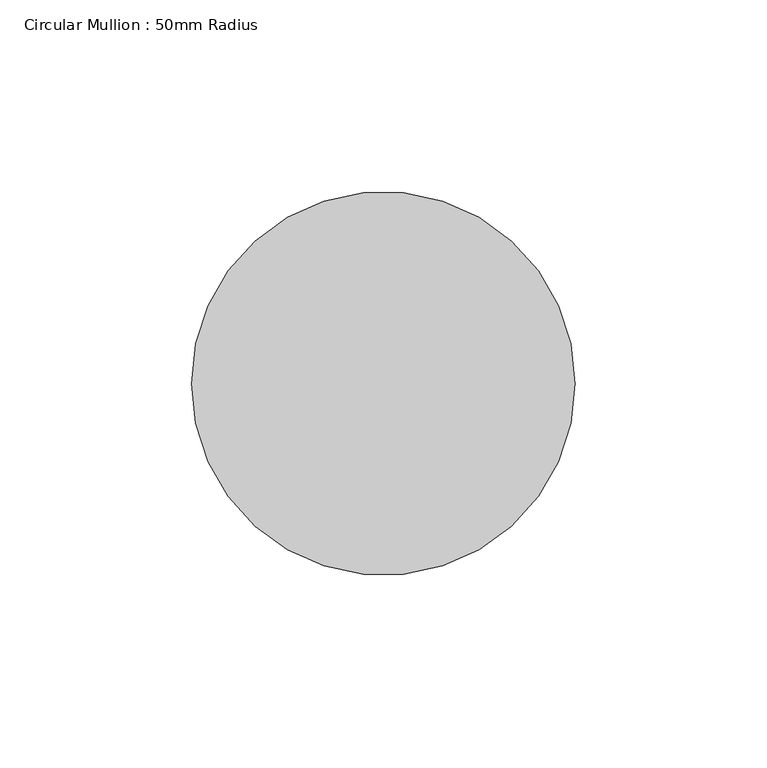
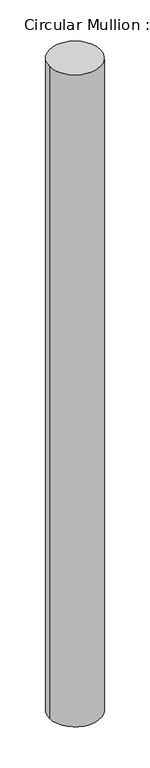
"""IFC4 building model written with IfcOpenShell, lengths in millimetres: member geometry, Circular Mullion : 50mm Radius."""

from ifc_helpers import new_model, si_unit, point, frame, origin, origin_2d, place, context, project, spatial, circle_curve, trimmed, segment, composite_curve, outline, extrude, source, transform, mapped, element, save


def circular_mullion_50mm_radius_b40ed272(model_context):
    return source(origin(), model_context, "Body", "SweptSolid", [
        extrude(outline(composite_curve([segment(trimmed(circle_curve(origin_2d(), 50.0), [point((50.0, 0.0))], [point((-50.0, 0.0))], False, "CARTESIAN"), True, "CONTINUOUS"), segment(trimmed(circle_curve(origin_2d(), 50.0), [point((-50.0, 0.0))], [point((50.0, 0.0))], False, "CARTESIAN"), True, "CONTINUOUS")], self_intersect=False)), frame((0.0, 0.0, -1351.6100393), z_axis=(0.0, 0.0, 1.0), x_axis=(1.0, 0.0, 0.0)), (0.0, 0.0, 1.0), 1351.6100393),
    ])


if __name__ == "__main__":
    model = new_model("IFC4")
    model_context = context("Model", 3, world=origin())
    ifc_project = project(units=[si_unit("LENGTHUNIT", "METRE", prefix="MILLI")], contexts=[model_context])
    site = spatial("IfcSite", under=ifc_project)
    building = spatial("IfcBuilding", under=site)
    placement = place(None, origin())
    circular_mullion_50mm_radius_shape = circular_mullion_50mm_radius_b40ed272(model_context)
    element("IfcMember", 1, ObjectType="Circular Mullion : 50mm Radius", at=placement, inside=building, context=model_context, shape_type="MappedRepresentation", body=[
        mapped(circular_mullion_50mm_radius_shape, transform((0.0, 0.0, 0.0), x_axis=(1.0, 0.0, 0.0), y_axis=(0.0, 1.0, 0.0), z_axis=(0.0, 0.0, 1.0))),
    ])
    save(model, "model.ifc")

# Revit data of these elements
# Type "Circular Mullion : 50mm Radius"
#   built-in parameter 1007350 = 0.164042 (stored number, unit not read)
# Element 1 (IfcMember, "Circular Mullion : 50mm Radius")
#   Materials on its faces: "Aluminium"
# Materials
#   "Aluminium": class "Metal", colour RGB 247 247 247, transparency 0, Description = "Aluminium 6061", Cost = 0
